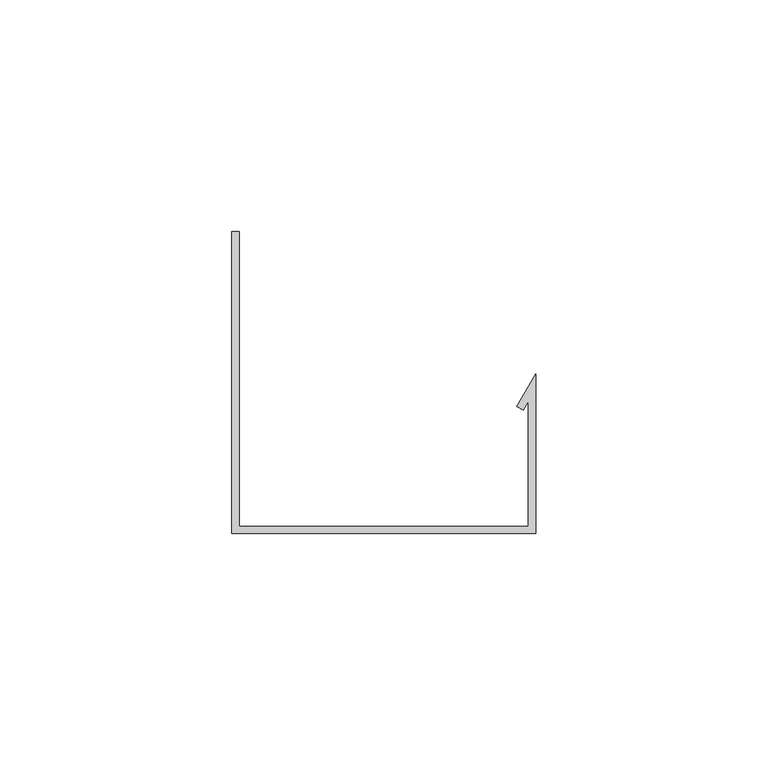
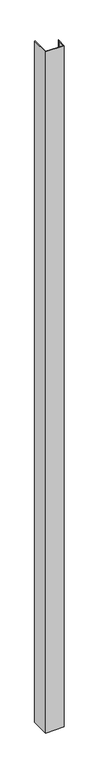
"""IFC4 building model written with IfcOpenShell, lengths in millimetres: proxy geometry, Generic Models 2:Generic Models 2:310765:Generic Models 2:310765 : Generic Models 2:Generic Models 2:310765:87 : Generic Models 2:Generic Models 2:310765:Generic Models 2:310765 : Generic Models 2:Generic Models 2:310765:300385."""

from ifc_helpers import new_model, si_unit, origin, origin_with_axes, place, context, project, spatial, polyline, outline, extrude, source, transform, mapped, element, save


def generic_models_7449f755(model_context):
    return source(origin(), model_context, "Body", "SweptSolid", [
        extrude(outline(polyline([(667550.0344867, -564675.7290364), (667550.0344867, -564610.6415364), (667551.6219867, -564610.6415364), (667551.6219867, -564674.1415364), (667613.8778802, -564674.1415364), (667613.8778802, -564647.1790235), (667612.7676476, -564649.1020028), (667611.3928322, -564648.3082528), (667615.4653802, -564641.2543929), (667615.4653802, -564675.7290364), (667550.0344867, -564675.7290364)])), origin_with_axes(), (0.0, 0.0, 1.0), 2508.9309299),
    ])


if __name__ == "__main__":
    model = new_model("IFC4")
    model_context = context("Model", 3, world=origin())
    ifc_project = project(units=[si_unit("LENGTHUNIT", "METRE", prefix="MILLI")], contexts=[model_context])
    site = spatial("IfcSite", under=ifc_project)
    building = spatial("IfcBuilding", under=site)
    placement = place(None, origin())
    generic_models_shape = generic_models_7449f755(model_context)
    element("IfcBuildingElementProxy", 1, Name="Generic Models 2:Generic Models 2:310765:Generic Models 2:310765 : Generic Models 2:Generic Models 2:310765:87 : Generic Models 2:Generic Models 2:310765:Generic Models 2:310765 : Generic Models 2:Generic Models 2:310765:300385", ObjectType="Generic Models 2:Generic Models 2:310765:Generic Models 2:310765 : Generic Models 2:Generic Models 2:310765:87 : Generic Models 2:Generic Models 2:310765:Generic Models 2:310765 : Generic Models 2:Generic Models 2:310765:300385", at=placement, inside=building, context=model_context, shape_type="MappedRepresentation", body=[
        mapped(generic_models_shape, transform((0.0, 0.0, 0.0), x_axis=(1.0, 0.0, 0.0), y_axis=(0.0, 1.0, 0.0), z_axis=(0.0, 0.0, 1.0))),
    ])
    save(model, "model.ifc")

# Revit data of these elements
# Type "Generic Models 2:Generic Models 2:310765:Generic Models 2:310765 : Generic Models 2:Generic Models 2:310765:87 : Generic Models 2:Generic Models 2:310765:Generic Models 2:310765 : Generic Models 2:Generic Models 2:310765:300385"
#   NameOverride = "Generic Models 2:Generic Models 2:310765:Generic Models 2:310765 : Generic Models 2:Generic Models 2:310765:300385"
#   ObjectTypeOverride = "Generic Models 2:310765 : Generic Models 2:Generic Models 2:310765"
#   Reference = "Generic Models 2"
#   Tag = "300385"
# Element 1 (IfcBuildingElementProxy, "Generic Models 2:Generic Models 2:310765:Generic Models 2:310765 : Generic Models 2:Generic Models 2:310765:87 : Generic Models 2:Generic Models 2:310765:Generic Models 2:310765 : Generic Models 2:Generic Models 2:310765:300385")
#   Materials on its faces: "JAMB TRIM"
# Materials
#   "JAMB TRIM": class "Unassigned", colour RGB 210 209 208, transparency 0, Cost = 0
